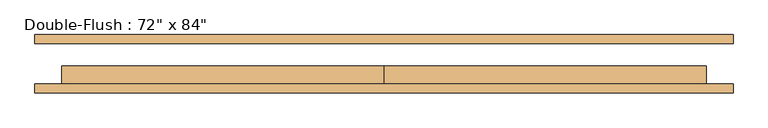
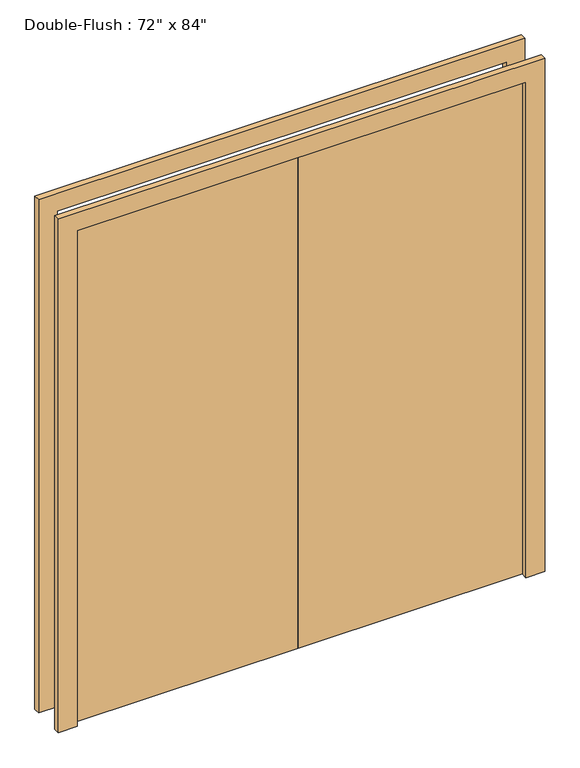
"""IFC4 building model written with IfcOpenShell, lengths in millimetres: door geometry."""

from ifc_helpers import new_model, si_unit, frame, origin, origin_with_axes, place, context, project, spatial, polyline, outline, extrude, source, transform, mapped, element, save


def door_5c6be3c9(model_context):
    return source(origin(), model_context, "Body", "SweptSolid", [
        extrude(outline(polyline([(0.0, -57.15), (0.0, -6.35), (914.4, -6.35), (914.4, -57.15), (0.0, -57.15)])), origin_with_axes(), (0.0, 0.0, 1.0), 2133.6),
        extrude(outline(polyline([(-914.4, -57.15), (-914.4, -6.35), (0.0, -6.35), (0.0, -57.15), (-914.4, -57.15)])), origin_with_axes(), (0.0, 0.0, 1.0), 2133.6),
        extrude(outline(polyline([(2133.6, -914.4), (2133.6, 914.4), (0.0, 914.4), (0.0, 990.6), (2209.8, 990.6), (2209.8, -990.6), (0.0, -990.6), (0.0, -914.4), (2133.6, -914.4)])), frame((0.0, 57.15, 0.0), z_axis=(0.0, 1.0, 0.0), x_axis=(0.0, 0.0, 1.0)), (0.0, 0.0, 1.0), 25.4),
        extrude(outline(polyline([(2133.6, -914.4), (2133.6, 914.4), (0.0, 914.4), (0.0, 990.6), (2209.8, 990.6), (2209.8, -990.6), (0.0, -990.6), (0.0, -914.4), (2133.6, -914.4)])), frame((0.0, -82.55, 0.0), z_axis=(0.0, 1.0, 0.0), x_axis=(0.0, 0.0, 1.0)), (0.0, 0.0, 1.0), 25.4),
    ])


if __name__ == "__main__":
    model = new_model("IFC4")
    model_context = context("Model", 3, world=origin())
    ifc_project = project(units=[si_unit("LENGTHUNIT", "METRE", prefix="MILLI")], contexts=[model_context])
    site = spatial("IfcSite", under=ifc_project)
    building = spatial("IfcBuilding", under=site)
    placement = place(None, origin())
    door_shape = door_5c6be3c9(model_context)
    element("IfcDoor", 1, ObjectType="Double-Flush : 72\" x 84\"", at=placement, inside=building, context=model_context, shape_type="MappedRepresentation", body=[
        mapped(door_shape, transform((0.0, 0.0, 0.0), x_axis=(1.0, 0.0, 0.0), y_axis=(0.0, 1.0, 0.0), z_axis=(0.0, 0.0, 1.0))),
    ])
    save(model, "model.ifc")

# Revit data of these elements
# Type "Double-Flush : 72\" x 84\""
#   Type Mark = "12"
#   Assembly Code = "C1020"
#   Thickness = 0' - 2"
#   Height = 7' - 0"
#   Trim Projection Ext = 0' - 1"
#   Trim Projection Int = 0' - 1"
#   Trim Width = 0' - 3"
#   Width = 6' - 0"
#   Function = 0
#   Door Material = Door - Panel
#   Frame Material = Door - Frame
#   Wall Closure = (empty or 0)
# Element 1 (IfcDoor, "Double-Flush : 72\" x 84\"")
#   Materials on its faces: "Door - Frame", "Door - Panel"
# Materials
#   "Door - Panel": class "Wood", colour RGB 210 159 95, transparency 0
#   "Door - Frame": class "Miscellaneous", colour RGB 118 70 51, transparency 0
